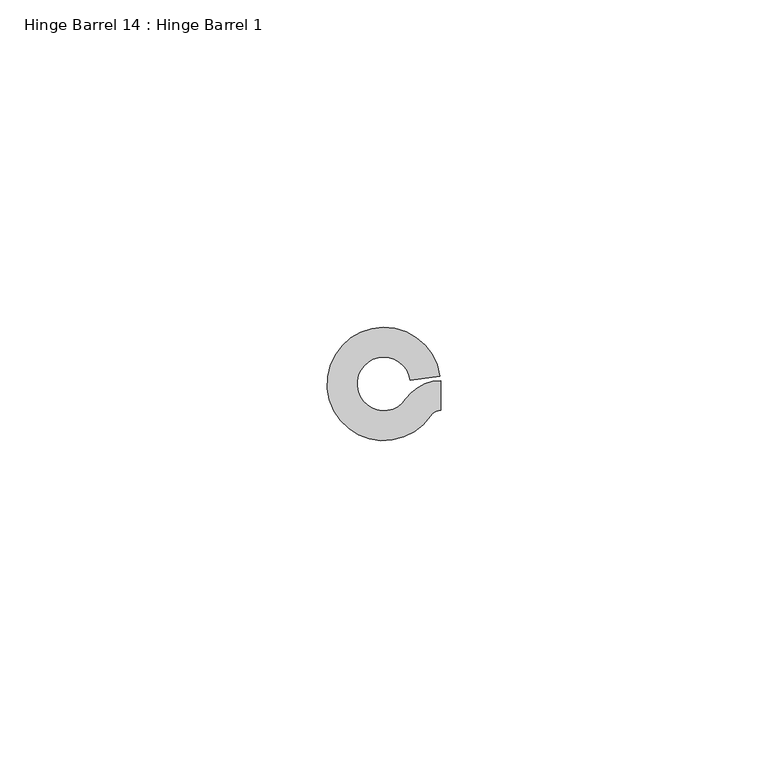
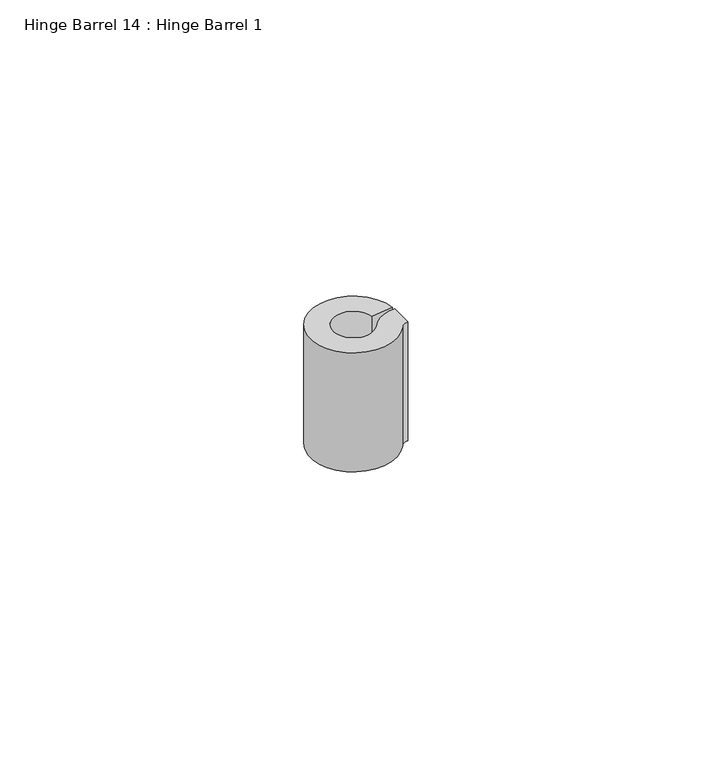
"""IFC4 building model written with IfcOpenShell, lengths in millimetres: proxy geometry, Hinge Barrel 14 : Hinge Barrel 1."""

import ifcopenshell
import ifcopenshell.guid

model = None  # the IFC model being written
_history = None  # IfcOwnerHistory: only IFC2X3 demands one
_inside = {}  # id of a spatial element -> (the spatial element, [elements in it])
_under = {}  # id of a project, library or spatial element -> (it, [spatial elements below it])
_declared = {}  # id of a project -> (the project, [libraries it declares])
_typed = {}  # id of a type object -> (the type object, [elements of that type])
_made_of = {}  # id of a material, layer set ... -> (it, [elements and type objects made of it])


def new_model(schema):
    """Start an empty IFC model of exactly this schema.

    Asked for "IFC4X3", IfcOpenShell would pick the latest addendum, in which some entities
    have other attributes; the version numbers below select the first issue.
    IFC2X3 requires an IfcOwnerHistory on every rooted entity: one is made here for all.
    """
    global model, _history
    if schema == "IFC4X3":
        model = ifcopenshell.file(schema_version=(4, 3, 0, 0))
    else:
        model = ifcopenshell.file(schema=schema)
    _inside.clear()
    _under.clear()
    _declared.clear()
    _typed.clear()
    _made_of.clear()
    _history = None
    if model.schema == "IFC2X3":
        org = make("IfcOrganization", Name="unknown")
        user = make(
            "IfcPersonAndOrganization",
            ThePerson=make("IfcPerson", FamilyName="unknown"),
            TheOrganization=org,
        )
        app = make(
            "IfcApplication",
            ApplicationDeveloper=org,
            Version="unknown",
            ApplicationFullName="unknown",
            ApplicationIdentifier="unknown",
        )
        _history = make(
            "IfcOwnerHistory",
            OwningUser=user,
            OwningApplication=app,
            ChangeAction="ADDED",
            CreationDate=0,
        )
    return model


def make(cls, **values):
    """One entity of the class cls with the attributes given. An attribute that is None is left unset."""
    return model.create_entity(
        cls, **{name: value for name, value in values.items() if value is not None}
    )


def rooted(cls, **values):
    """An entity with a GlobalId (a new one), such as an element, a storey or a relation."""
    return make(cls, GlobalId=ifcopenshell.guid.new(), OwnerHistory=_history, **values)


def si_unit(unit_type, name, prefix=None):
    """IfcSIUnit, for example si_unit("LENGTHUNIT", "METRE", prefix="MILLI")."""
    return make("IfcSIUnit", UnitType=unit_type, Prefix=prefix, Name=name)


def assignment(units):
    """IfcUnitAssignment: the units of a project."""
    return None if units is None else make("IfcUnitAssignment", Units=units)


def point(xyz):
    """IfcCartesianPoint."""
    return None if xyz is None else make("IfcCartesianPoint", Coordinates=xyz)


def direction(xyz):
    """IfcDirection."""
    return None if xyz is None else make("IfcDirection", DirectionRatios=xyz)


def frame(location, z_axis=None, x_axis=None):
    """IfcAxis2Placement3D, a coordinate frame: its origin and axes. An axis left out is left unset."""
    return make(
        "IfcAxis2Placement3D",
        Location=point(location),
        Axis=direction(z_axis),
        RefDirection=direction(x_axis),
    )


def frame_2d(location, x_axis=None):
    """IfcAxis2Placement2D, a coordinate frame in the plane: its origin and x axis."""
    return make(
        "IfcAxis2Placement2D", Location=point(location), RefDirection=direction(x_axis)
    )


def origin():
    """The frame at (0, 0, 0) with its axes left unset."""
    return frame((0.0, 0.0, 0.0))


def place(relative_to, where):
    """IfcLocalPlacement: puts the frame where relative to a parent placement (None: the world)."""
    return make(
        "IfcLocalPlacement", PlacementRelTo=relative_to, RelativePlacement=where
    )


def context(
    kind, dimensions, precision=None, world=None, true_north=None, identifier=None
):
    """IfcGeometricRepresentationContext, for example the 3D "Model" context."""
    return make(
        "IfcGeometricRepresentationContext",
        ContextIdentifier=identifier,
        ContextType=kind,
        CoordinateSpaceDimension=dimensions,
        Precision=precision,
        WorldCoordinateSystem=world,
        TrueNorth=true_north,
    )


def project(units=None, contexts=None):
    """IfcProject with its units and contexts."""
    return rooted(
        "IfcProject",
        Name="project",
        RepresentationContexts=contexts,
        UnitsInContext=assignment(units),
    )


def spatial(cls, under=None, at=None, **own):
    """A site, building, storey or space (cls), placed at a placement, below another one or the project."""
    s = rooted(cls, ObjectPlacement=at, **own)
    if under is not None:
        _under.setdefault(under.id(), (under, []))[1].append(s)
    return s


def polyline(points):
    """IfcPolyline through the points."""
    return make("IfcPolyline", Points=[point(p) for p in points])


def circle_curve(where, radius):
    """IfcCircle in the frame where."""
    return make("IfcCircle", Position=where, Radius=radius)


def trimmed(basis, trim1, trim2, sense, master):
    """IfcTrimmedCurve: the piece of a basis curve between two trims."""
    return make(
        "IfcTrimmedCurve",
        BasisCurve=basis,
        Trim1=trim1,
        Trim2=trim2,
        SenseAgreement=sense,
        MasterRepresentation=master,
    )


def segment(curve, same_sense, transition):
    """IfcCompositeCurveSegment."""
    return make(
        "IfcCompositeCurveSegment",
        Transition=transition,
        SameSense=same_sense,
        ParentCurve=curve,
    )


def composite_curve(segments, self_intersect=None):
    """IfcCompositeCurve: segments joined end to end."""
    return make("IfcCompositeCurve", Segments=segments, SelfIntersect=self_intersect)


def outline(outer, holes=None, kind="AREA"):
    """IfcArbitraryClosedProfileDef: a profile drawn as a closed curve; with holes, ...WithVoids."""
    if holes is None:
        return make("IfcArbitraryClosedProfileDef", ProfileType=kind, OuterCurve=outer)
    return make(
        "IfcArbitraryProfileDefWithVoids",
        ProfileType=kind,
        OuterCurve=outer,
        InnerCurves=holes,
    )


def extrude(swept, where, along, depth):
    """IfcExtrudedAreaSolid: the profile swept, set in the frame where, extruded along a direction by depth."""
    return make(
        "IfcExtrudedAreaSolid",
        SweptArea=swept,
        Position=where,
        ExtrudedDirection=direction(along),
        Depth=depth,
    )


def shape(context_of_items, identifier, shape_type, items):
    """IfcShapeRepresentation: the items that make up one representation, for example the "Body"."""
    return make(
        "IfcShapeRepresentation",
        ContextOfItems=context_of_items,
        RepresentationIdentifier=identifier,
        RepresentationType=shape_type,
        Items=items,
    )


def source(mapping_origin, context_of_items, identifier, shape_type, items):
    """IfcRepresentationMap: a shape defined once, which mapped items show again and again."""
    return make(
        "IfcRepresentationMap",
        MappingOrigin=mapping_origin,
        MappedRepresentation=shape(context_of_items, identifier, shape_type, items),
    )


def transform(
    local_origin,
    x_axis=None,
    y_axis=None,
    z_axis=None,
    scale=None,
    scale2=None,
    scale3=None,
    uniform=True,
):
    """IfcCartesianTransformationOperator3D, or its non-uniform kind. x_axis, y_axis, z_axis: its Axis1, 2, 3."""
    if uniform:
        return make(
            "IfcCartesianTransformationOperator3D",
            Axis1=direction(x_axis),
            Axis2=direction(y_axis),
            LocalOrigin=point(local_origin),
            Scale=scale,
            Axis3=direction(z_axis),
        )
    return make(
        "IfcCartesianTransformationOperator3DnonUniform",
        Axis1=direction(x_axis),
        Axis2=direction(y_axis),
        LocalOrigin=point(local_origin),
        Scale=scale,
        Axis3=direction(z_axis),
        Scale2=scale2,
        Scale3=scale3,
    )


def mapped(mapping_source, mapping_target):
    """IfcMappedItem: shows the shape of a source again, moved by a transform."""
    return make(
        "IfcMappedItem", MappingSource=mapping_source, MappingTarget=mapping_target
    )


def made_of(thing, what):
    """Note that an element or type object is made of a material, layer set ...; save() writes the relation."""
    if what is not None:
        _made_of.setdefault(what.id(), (what, []))[1].append(thing)
    return thing


def element(
    cls,
    number,
    at=None,
    inside=None,
    cuts=None,
    type_object=None,
    material=None,
    context=None,
    identifier="Body",
    shape_type=None,
    held_by="IfcProductDefinitionShape",
    body=None,
    shapes=None,
    **own,
):
    """One element of the class cls, such as IfcWall. Its Tag is "e" and its number.

    at: its placement. inside: the storey or other place that contains it. cuts: it is an
    opening in that element (IfcRelVoidsElement). A single representation is given by context,
    identifier, shape_type and body (its items); several are given by shapes. held_by: the class
    of the entity that holds the representations. save() writes the other relations.
    """
    e = rooted(cls, Tag="e%d" % number, ObjectPlacement=at, **own)
    if body is not None:
        shapes = [shape(context, identifier, shape_type, body)]
    if shapes is not None:
        e.Representation = make(held_by, Representations=shapes)
    if inside is not None:
        _inside.setdefault(inside.id(), (inside, []))[1].append(e)
    if cuts is not None:
        rooted(
            "IfcRelVoidsElement", RelatingBuildingElement=cuts, RelatedOpeningElement=e
        )
    if type_object is not None:
        _typed.setdefault(type_object.id(), (type_object, []))[1].append(e)
    return made_of(e, material)


def aggregate(whole, parts):
    """IfcRelAggregates: a whole, such as a stair, and the parts it consists of."""
    return rooted("IfcRelAggregates", RelatingObject=whole, RelatedObjects=parts)


def save(model, path):
    """Write the relations noted so far, then the file.

    IfcRelAggregates (storeys below a building ...), IfcRelContainedInSpatialStructure (elements
    in a storey), IfcRelDefinesByType, IfcRelAssociatesMaterial and IfcRelDeclares: one each for
    every whole, place, type object, material and project.
    """
    for whole, parts in _under.values():
        aggregate(whole, parts)
    for where, things in _inside.values():
        rooted(
            "IfcRelContainedInSpatialStructure",
            RelatedElements=things,
            RelatingStructure=where,
        )
    for kind, things in _typed.values():
        rooted("IfcRelDefinesByType", RelatedObjects=things, RelatingType=kind)
    for what, things in _made_of.values():
        rooted("IfcRelAssociatesMaterial", RelatedObjects=things, RelatingMaterial=what)
    for by, libraries in _declared.values():
        rooted("IfcRelDeclares", RelatingContext=by, RelatedDefinitions=libraries)
    model.write(path)


def hinge_barrel_14_hinge_barrel_1_75b3f5ff(model_context):
    return source(origin(), model_context, "Body", "SweptSolid", [
        extrude(outline(composite_curve([segment(trimmed(circle_curve(frame_2d((587327.8245257, -533990.5568067)), 6.4044851), [point((587322.5194669, -533986.9688017))], [point((587327.8245257, -533984.1523216))], False, "CARTESIAN"), True, "CONTINUOUS"), segment(polyline([(587327.8245257, -533984.1523216), (587327.8245257, -533988.7163841)]), True, "CONTINUOUS"), segment(trimmed(circle_curve(frame_2d((587327.8245257, -533990.5568067)), 1.8404226), [point((587327.8245257, -533988.7163841))], [point((587326.3000393, -533989.5257409))], True, "CARTESIAN"), True, "CONTINUOUS"), segment(trimmed(circle_curve(frame_2d((587319.1320739, -533984.6777841)), 8.6534625), [point((587326.3000393, -533989.5257409))], [point((587327.7022899, -533983.4803654))], False, "CARTESIAN"), True, "CONTINUOUS"), segment(polyline([(587327.7022899, -533983.4803654), (587323.1821338, -533984.1119153)]), True, "CONTINUOUS"), segment(trimmed(circle_curve(frame_2d((587319.1320739, -533984.6777841)), 4.0894), [point((587323.1821338, -533984.1119153))], [point((587322.5194669, -533986.9688017))], True, "CARTESIAN"), True, "CONTINUOUS")], self_intersect=False)), frame((0.0, 0.0, 336.55), z_axis=(0.0, 0.0, 1.0), x_axis=(1.0, 0.0, 0.0)), (0.0, 0.0, 1.0), 25.4),
    ])


if __name__ == "__main__":
    model = new_model("IFC4")
    model_context = context("Model", 3, world=origin())
    ifc_project = project(units=[si_unit("LENGTHUNIT", "METRE", prefix="MILLI")], contexts=[model_context])
    site = spatial("IfcSite", under=ifc_project)
    building = spatial("IfcBuilding", under=site)
    placement = place(None, origin())
    hinge_barrel_14_hinge_barrel_1_shape = hinge_barrel_14_hinge_barrel_1_75b3f5ff(model_context)
    element("IfcBuildingElementProxy", 1, Name="Hinge Barrel 14 : Hinge Barrel 1", ObjectType="Hinge Barrel 14 : Hinge Barrel 1", at=placement, inside=building, context=model_context, shape_type="MappedRepresentation", body=[
        mapped(hinge_barrel_14_hinge_barrel_1_shape, transform((0.0, 0.0, 0.0), x_axis=(1.0, 0.0, 0.0), y_axis=(0.0, 1.0, 0.0), z_axis=(0.0, 0.0, 1.0))),
    ])
    save(model, "model.ifc")

# Revit data of these elements
# Element 1 (IfcBuildingElementProxy, "Hinge Barrel 14 : Hinge Barrel 1")
#   Materials on its faces: "6\"X6\" WELD-ON STL BUTT HINGE"
# Materials
#   "6\"X6\" WELD-ON STL BUTT HINGE": class "Metal", colour RGB 189 187 185, transparency 0, Description = "Carbon steel", Cost = 0
